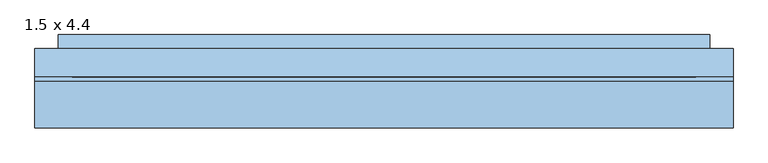
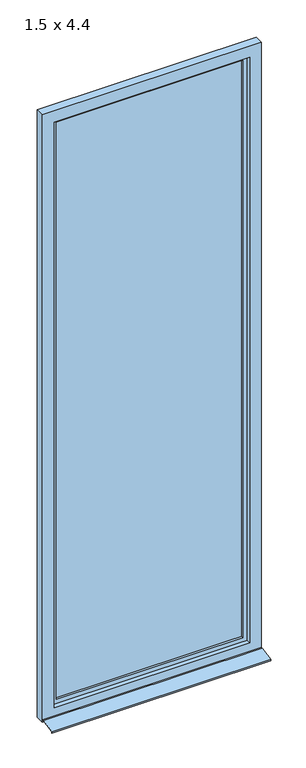
"""IFC4 building model written with IfcOpenShell, lengths in millimetres: window geometry, Fenstertür 1-flg : 1.5 x 4.4."""

from ifc_helpers import new_model, si_unit, frame, origin, place, context, project, spatial, polyline, outline, extrude, faceted_brep, source, transform, mapped, element, save


def window_1_5_x_4_4_3b2dc675(model_context):
    return source(origin(), model_context, "Body", "SolidModel", [
        extrude(outline(polyline([(4400.0, 750.0), (4400.0, -750.0), (0.0, -750.0), (0.0, 750.0), (4400.0, 750.0)]), holes=[polyline([(4320.0, 670.0), (80.0, 670.0), (80.0, -670.0), (4320.0, -670.0), (4320.0, 670.0)])]), frame((0.0, -120.0, 0.0), z_axis=(0.0, 1.0, 0.0), x_axis=(0.0, 0.0, 1.0)), (0.0, 0.0, 1.0), 60.0),
        faceted_brep([(700.0, -60.0, 4350.0), (700.0, -60.0, 50.0), (700.0, -30.0, 50.0), (700.0, -30.0, 4350.0), (-700.0, -30.0, 50.0), (-700.0, -30.0, 4350.0), (640.0, -30.0, 110.0), (640.0, -30.0, 4290.0), (-640.0, -30.0, 4290.0), (-640.0, -30.0, 110.0), (-700.0, -60.0, 50.0), (-700.0, -60.0, 4350.0), (670.0, -60.0, 4320.0), (670.0, -60.0, 80.0), (-670.0, -60.0, 80.0), (-670.0, -60.0, 4320.0), (670.0, -90.0, 4320.0), (670.0, -90.0, 80.0), (-670.0, -90.0, 80.0), (-670.0, -90.0, 4320.0), (640.0, -90.0, 4290.0), (640.0, -90.0, 110.0), (-640.0, -90.0, 110.0), (-640.0, -90.0, 4290.0)], [[[0, 1, 2, 3]], [[3, 2, 4, 5], [6, 7, 8, 9]], [[1, 10, 4, 2]], [[1, 0, 11, 10], [12, 13, 14, 15]], [[16, 17, 13, 12]], [[17, 18, 14, 13]], [[17, 16, 19, 18], [20, 21, 22, 23]], [[7, 6, 21, 20]], [[6, 9, 22, 21]], [[10, 11, 5, 4]], [[18, 19, 15, 14]], [[9, 8, 23, 22]], [[11, 0, 3, 5]], [[19, 16, 12, 15]], [[8, 7, 20, 23]]]),
        extrude(outline(polyline([(-130.0221543, 20.0), (-120.0, 20.0), (-120.0, 18.0), (-129.8240723, 18.0), (-228.0, -1.6395366), (-228.0, -10.0), (-230.0, -10.0), (-230.0, 0.0), (-130.0221543, 20.0)])), frame((-750.0, 0.0, 0.0), z_axis=(1.0, 0.0, 0.0), x_axis=(0.0, 1.0, 0.0)), (0.0, 0.0, 1.0), 1500.0),
        extrude(outline(polyline([(640.0, -45.0), (640.0, -75.0), (-640.0, -75.0), (-640.0, -45.0), (640.0, -45.0)])), frame((0.0, 0.0, 110.0), z_axis=(0.0, 0.0, 1.0), x_axis=(1.0, 0.0, 0.0)), (0.0, 0.0, 1.0), 4180.0),
    ])


if __name__ == "__main__":
    model = new_model("IFC4")
    model_context = context("Model", 3, world=origin())
    ifc_project = project(units=[si_unit("LENGTHUNIT", "METRE", prefix="MILLI")], contexts=[model_context])
    site = spatial("IfcSite", under=ifc_project)
    building = spatial("IfcBuilding", under=site)
    placement = place(None, origin())
    window_1_5_x_4_4_shape = window_1_5_x_4_4_3b2dc675(model_context)
    element("IfcWindow", 1, ObjectType="Fenstertür 1-flg : 1.5 x 4.4", at=placement, inside=building, context=model_context, shape_type="MappedRepresentation", body=[
        mapped(window_1_5_x_4_4_shape, transform((0.0, 0.0, 0.0), x_axis=(1.0, 0.0, 0.0), y_axis=(0.0, 1.0, 0.0), z_axis=(0.0, 0.0, 1.0))),
    ])
    save(model, "model.ifc")

# Revit data of these elements
# Type "Fenstertür 1-flg : 1.5 x 4.4"
#   Type Mark = "58"
#   Operation = "SinglePanel"
#   Construction Type Id = "GSP4R"
#   Keynote = "16.05.01"
#   Analytic Construction = "1/8 Zoll Pilkington-Verglasung einfach"
#   Visual Light Transmittance = 0.9
#   Thermal Resistance (R) = 0.1491 (m²·K)/W
#   Solar Heat Gain Coefficient = 0.86
#   Rough Width = 1.500 m
#   Rough Height = 4.400 m
#   Heat Transfer Coefficient (U) = 6.7069 W/(m²·K)
#   Rahmentiefe = 0.060 m
#   Rahmenhöhe - unten = 0.080 m
#   Rahmenhöhe - oben = 0.080 m
#   Rahmenbreite = 0.080 m
#   Height = 4.400 m
#   Tiefe Flügel = 0.060 m
#   Flügelbreite = 0.060 m
#   Einbautiefe (von außen) [instance default] = 0.080 m
#   Width = 1.500 m
#   Kippflügel [instance default] = yes
#   Drehflügel im Grundriss darstellen [instance default] = yes
#   Drehflügel 1 [instance default] = yes
#   Rahmen 1 [instance default] = none
#   Glas [instance default] = none
#   Flügel [instance default] = none
#   Fensterbank Außenseite [instance default] = none
#   Wall Closure = (empty or 0)
# Element 1 (IfcWindow, "Fenstertür 1-flg : 1.5 x 4.4")
#   Materials on its faces: "Kunststoff - Weiß", "Glas"
# Materials
#   "Kunststoff - Weiß": class "Kunststoff", colour RGB 249 249 249, transparency 0, Cost = 0
#   "Glas": class "Glas", colour RGB 0 0 255, transparency 0.75, Comments = "Render-Darstellung nicht aktualisiert ", Cost = 0
